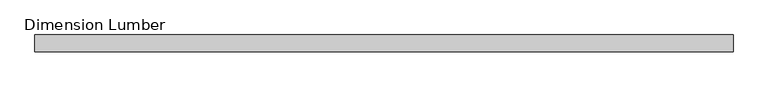
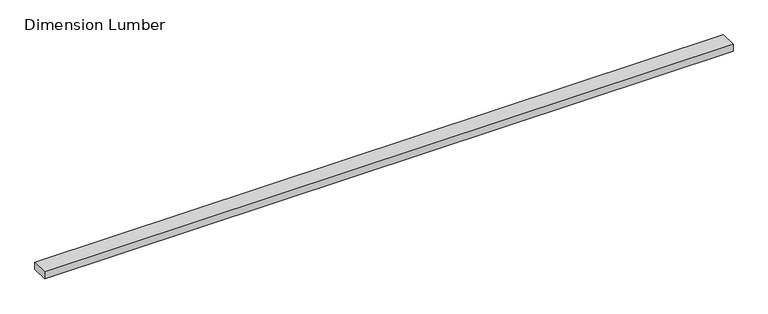
"""IFC4 building model written with IfcOpenShell, lengths in millimetres: beam geometry, Dimension Lumber : Top Supporting Lumbers."""

from ifc_helpers import new_model, si_unit, frame, origin, place, context, project, spatial, polyline, outline, extrude, source, transform, mapped, element, save


def dimension_lumber_e331b447(model_context):
    return source(origin(), model_context, "Body", "SweptSolid", [
        extrude(outline(polyline([(1838.325, 44.45), (1838.325, -44.45), (-1838.325, -44.45), (-1838.325, 44.45), (1838.325, 44.45)])), frame((0.0, 0.0, -19.05), z_axis=(0.0, 0.0, 1.0), x_axis=(1.0, 0.0, 0.0)), (0.0, 0.0, 1.0), 38.1),
    ])


if __name__ == "__main__":
    model = new_model("IFC4")
    model_context = context("Model", 3, world=origin())
    ifc_project = project(units=[si_unit("LENGTHUNIT", "METRE", prefix="MILLI")], contexts=[model_context])
    site = spatial("IfcSite", under=ifc_project)
    building = spatial("IfcBuilding", under=site)
    placement = place(None, origin())
    dimension_lumber_shape = dimension_lumber_e331b447(model_context)
    element("IfcBeam", 1, ObjectType="Dimension Lumber : Top Supporting Lumbers", at=placement, inside=building, context=model_context, shape_type="MappedRepresentation", body=[
        mapped(dimension_lumber_shape, transform((0.0, 0.0, 0.0), x_axis=(1.0, 0.0, 0.0), y_axis=(0.0, 1.0, 0.0), z_axis=(0.0, 0.0, 1.0))),
    ])
    save(model, "model.ifc")

# Revit data of these elements
# Type "Dimension Lumber : Top Supporting Lumbers"
#   Assembly Code = "B10"
#   A = 0.0364583 SF
#   Length [instance default] = 5' - 0"
#   b = 0' - 3 1/2"
#   d = 0' - 1 1/2"
#   Structural Material [instance default] = Softwood, Lumber
# Element 1 (IfcBeam, "Dimension Lumber : Top Supporting Lumbers")
#   Structural Material = Douglas Fir #2
#   Materials on its faces: "Douglas Fir #2"
# Materials
#   "Softwood, Lumber": class "Wood", colour RGB 223 192 134, transparency 0, Description = "Pinus Echinata", Cost = 0
#   "Douglas Fir #2": class "Wood", colour RGB 223 192 134, transparency 0, Description = "Pinus Echinata", Cost = 0
